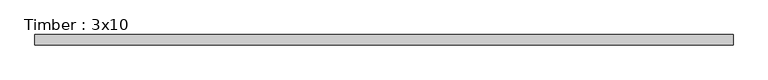
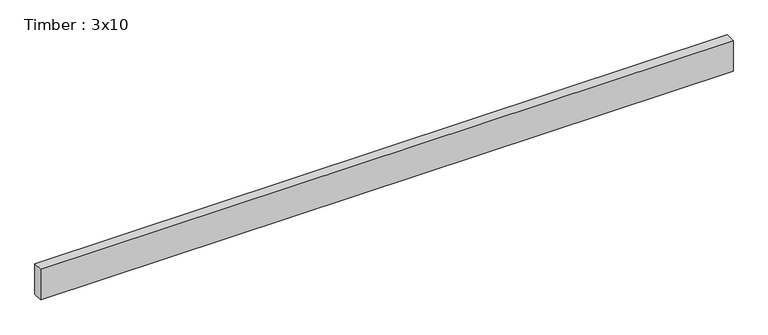
"""IFC4 building model written with IfcOpenShell, lengths in millimetres: beam geometry, Timber : 3x10."""

from ifc_helpers import new_model, si_unit, frame, origin, place, context, project, spatial, polyline, outline, extrude, source, transform, mapped, element, save


def timber_3x10_eec112f8(model_context):
    return source(origin(), model_context, "Body", "SweptSolid", [
        extrude(outline(polyline([(2565.4, 38.1), (2565.4, -38.1), (-2641.6, -38.1), (-2641.6, 38.1), (2565.4, 38.1)])), frame((0.0, 0.0, -120.65), z_axis=(0.0, 0.0, 1.0), x_axis=(1.0, 0.0, 0.0)), (0.0, 0.0, 1.0), 241.3),
    ])


if __name__ == "__main__":
    model = new_model("IFC4")
    model_context = context("Model", 3, world=origin())
    ifc_project = project(units=[si_unit("LENGTHUNIT", "METRE", prefix="MILLI")], contexts=[model_context])
    site = spatial("IfcSite", under=ifc_project)
    building = spatial("IfcBuilding", under=site)
    placement = place(None, origin())
    timber_3x10_shape = timber_3x10_eec112f8(model_context)
    element("IfcBeam", 1, ObjectType="Timber : 3x10", at=placement, inside=building, context=model_context, shape_type="MappedRepresentation", body=[
        mapped(timber_3x10_shape, transform((0.0, 0.0, 0.0), x_axis=(1.0, 0.0, 0.0), y_axis=(0.0, 1.0, 0.0), z_axis=(0.0, 0.0, 1.0))),
    ])
    save(model, "model.ifc")

# Revit data of these elements
# Type "Timber : 3x10"
#   Assembly Code = "B10"
#   A = 0.362847 SF
#   Length [instance default] = 5' - 0"
#   b = 0' - 3"
#   d = 0' - 9 1/2"
#   Structural Material [instance default] = Softwood, Lumber
# Element 1 (IfcBeam, "Timber : 3x10")
#   Materials on its faces: "Softwood, Lumber"
# Materials
#   "Softwood, Lumber": class "Wood", colour RGB 144 113 62, transparency 0, Description = "Pinus Echinata", Cost = 0
